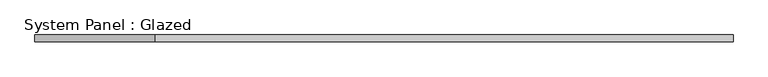
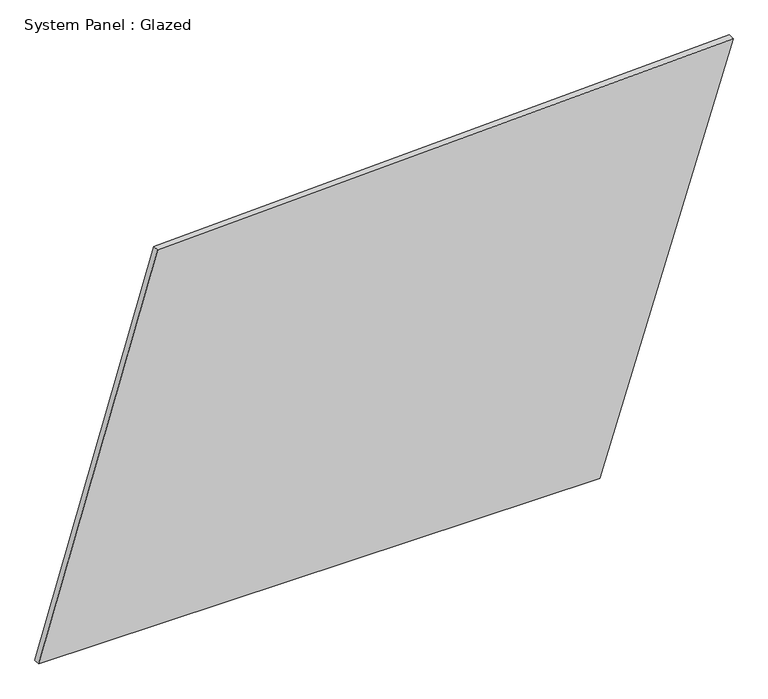
"""IFC4 building model written with IfcOpenShell, lengths in millimetres: plate geometry, System Panel : Glazed."""

from ifc_helpers import new_model, si_unit, frame, origin, place, context, project, spatial, polyline, outline, extrude, source, transform, mapped, element, save


def system_panel_glazed_e8d51dbd(model_context):
    return source(origin(), model_context, "Body", "SweptSolid", [
        extrude(outline(polyline([(0.0, -1318.8454955), (0.0, 811.5418879), (1589.2531484, 1318.8454955), (1504.2255239, -866.8369541), (0.0, -1318.8454955)])), frame((0.0, -49.5, 0.0), z_axis=(0.0, 1.0, 0.0), x_axis=(0.0, 0.0, 1.0)), (0.0, 0.0, 1.0), 25.0),
    ])


if __name__ == "__main__":
    model = new_model("IFC4")
    model_context = context("Model", 3, world=origin())
    ifc_project = project(units=[si_unit("LENGTHUNIT", "METRE", prefix="MILLI")], contexts=[model_context])
    site = spatial("IfcSite", under=ifc_project)
    building = spatial("IfcBuilding", under=site)
    placement = place(None, origin())
    system_panel_glazed_shape = system_panel_glazed_e8d51dbd(model_context)
    element("IfcPlate", 1, ObjectType="System Panel : Glazed", at=placement, inside=building, context=model_context, shape_type="MappedRepresentation", body=[
        mapped(system_panel_glazed_shape, transform((0.0, 0.0, 0.0), x_axis=(1.0, 0.0, 0.0), y_axis=(0.0, 1.0, 0.0), z_axis=(0.0, 0.0, 1.0))),
    ])
    save(model, "model.ifc")

# Revit data of these elements
# Element 1 (IfcPlate, "System Panel : Glazed")
#   Materials on its faces: "Glass, Clear Glazing"
# Materials
#   "Glass, Clear Glazing": class "Glass", colour RGB 247 249 248, transparency 0.85, Description = "Clear glazing", Cost = 0
